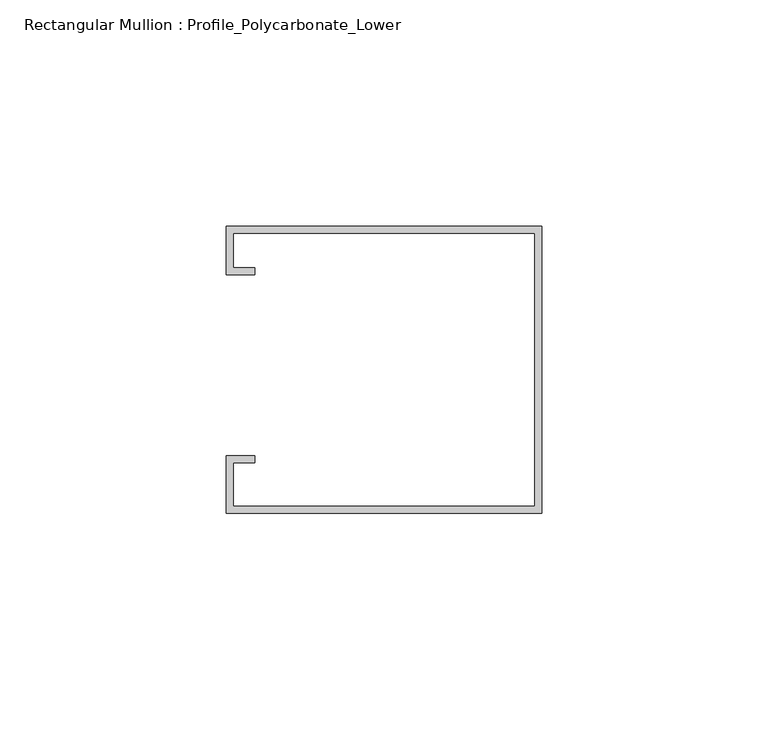
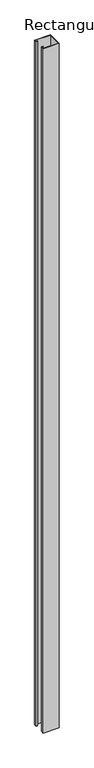
"""IFC4 building model written with IfcOpenShell, lengths in millimetres: member geometry, Rectangular Mullion : Profile_Polycarbonate_Lower."""

from ifc_helpers import new_model, si_unit, frame, origin, place, context, project, spatial, polyline, outline, extrude, source, transform, mapped, element, save


def rectangular_mullion_profile_polycarbonate_lower_46d97ac2(model_context):
    return source(origin(), model_context, "Body", "SweptSolid", [
        extrude(outline(polyline([(0.0, -32.7), (-69.85, -32.7), (-69.85, -20.0), (-63.5, -20.0), (-63.5, -21.5875), (-68.2625, -21.5875), (-68.2625, -31.1125), (-1.5875, -31.1125), (-1.5875, 29.2125), (-68.2625, 29.2125), (-68.2625, 21.5875), (-63.5, 21.5875), (-63.5, 20.0), (-69.85, 20.0), (-69.85, 30.8), (0.0, 30.8), (0.0, -32.7)])), frame((0.0, 0.0, -3149.6), z_axis=(0.0, 0.0, 1.0), x_axis=(1.0, 0.0, 0.0)), (0.0, 0.0, 1.0), 3149.6),
    ])


if __name__ == "__main__":
    model = new_model("IFC4")
    model_context = context("Model", 3, world=origin())
    ifc_project = project(units=[si_unit("LENGTHUNIT", "METRE", prefix="MILLI")], contexts=[model_context])
    site = spatial("IfcSite", under=ifc_project)
    building = spatial("IfcBuilding", under=site)
    placement = place(None, origin())
    rectangular_mullion_profile_polycarbonate_lower_shape = rectangular_mullion_profile_polycarbonate_lower_46d97ac2(model_context)
    element("IfcMember", 1, ObjectType="Rectangular Mullion : Profile_Polycarbonate_Lower", at=placement, inside=building, context=model_context, shape_type="MappedRepresentation", body=[
        mapped(rectangular_mullion_profile_polycarbonate_lower_shape, transform((0.0, 0.0, 0.0), x_axis=(1.0, 0.0, 0.0), y_axis=(0.0, 1.0, 0.0), z_axis=(0.0, 0.0, 1.0))),
    ])
    save(model, "model.ifc")

# Revit data of these elements
# Type "Rectangular Mullion : Profile_Polycarbonate_Lower"
#   built-in parameter 1007322 = 0.208333 (stored number, unit not read)
#   built-in parameter 1007321 = 0 (stored number, unit not read)
#   built-in parameter 1007320 = 0.00520833 (stored number, unit not read)
# Element 1 (IfcMember, "Rectangular Mullion : Profile_Polycarbonate_Lower")
#   Materials on its faces: "ALUMINUM PROFILE AT POLYCARBONATE PANEL"
# Materials
#   "ALUMINUM PROFILE AT POLYCARBONATE PANEL": class "Metal", colour RGB 244 244 244, transparency 0, Description = "Aluminum 6061", Cost = 0
